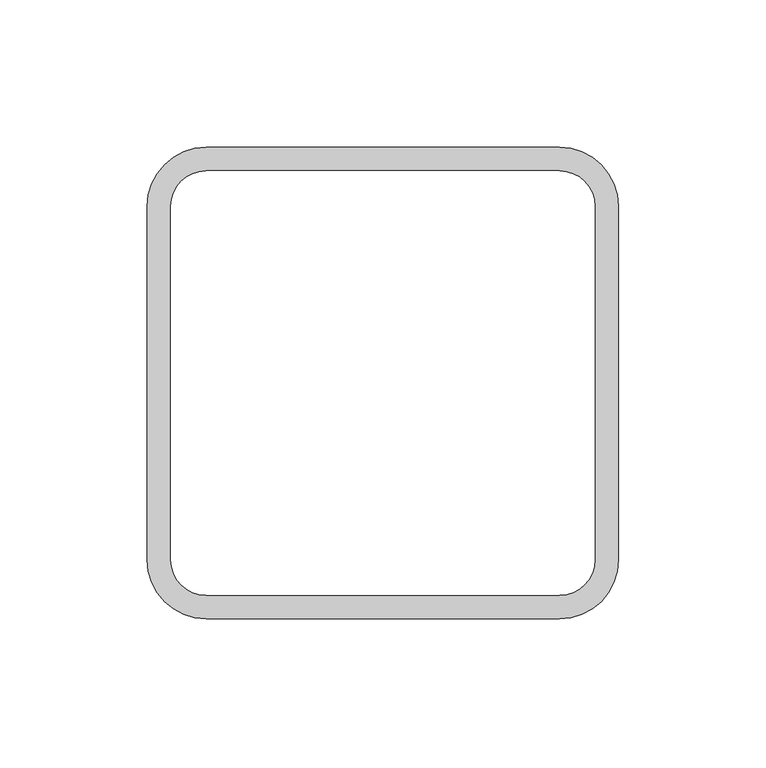
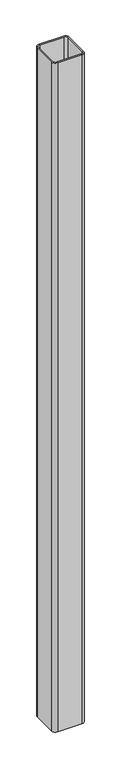
"""IFC4 building model written with IfcOpenShell, lengths in millimetres: column geometry, NLRS_28_SCO_TLB_stalen kolom buisprofiel koudgevormd vierkant-BCPG-MMBS-SRP_gen_rsf : stalen kolom buisprofiel koudgevormd vierkant RHSC_gen__160x160x8."""

import ifcopenshell
import ifcopenshell.guid

model = None  # the IFC model being written
_history = None  # IfcOwnerHistory: only IFC2X3 demands one
_inside = {}  # id of a spatial element -> (the spatial element, [elements in it])
_under = {}  # id of a project, library or spatial element -> (it, [spatial elements below it])
_declared = {}  # id of a project -> (the project, [libraries it declares])
_typed = {}  # id of a type object -> (the type object, [elements of that type])
_made_of = {}  # id of a material, layer set ... -> (it, [elements and type objects made of it])


def new_model(schema):
    """Start an empty IFC model of exactly this schema.

    Asked for "IFC4X3", IfcOpenShell would pick the latest addendum, in which some entities
    have other attributes; the version numbers below select the first issue.
    IFC2X3 requires an IfcOwnerHistory on every rooted entity: one is made here for all.
    """
    global model, _history
    if schema == "IFC4X3":
        model = ifcopenshell.file(schema_version=(4, 3, 0, 0))
    else:
        model = ifcopenshell.file(schema=schema)
    _inside.clear()
    _under.clear()
    _declared.clear()
    _typed.clear()
    _made_of.clear()
    _history = None
    if model.schema == "IFC2X3":
        org = make("IfcOrganization", Name="unknown")
        user = make(
            "IfcPersonAndOrganization",
            ThePerson=make("IfcPerson", FamilyName="unknown"),
            TheOrganization=org,
        )
        app = make(
            "IfcApplication",
            ApplicationDeveloper=org,
            Version="unknown",
            ApplicationFullName="unknown",
            ApplicationIdentifier="unknown",
        )
        _history = make(
            "IfcOwnerHistory",
            OwningUser=user,
            OwningApplication=app,
            ChangeAction="ADDED",
            CreationDate=0,
        )
    return model


def make(cls, **values):
    """One entity of the class cls with the attributes given. An attribute that is None is left unset."""
    return model.create_entity(
        cls, **{name: value for name, value in values.items() if value is not None}
    )


def rooted(cls, **values):
    """An entity with a GlobalId (a new one), such as an element, a storey or a relation."""
    return make(cls, GlobalId=ifcopenshell.guid.new(), OwnerHistory=_history, **values)


def si_unit(unit_type, name, prefix=None):
    """IfcSIUnit, for example si_unit("LENGTHUNIT", "METRE", prefix="MILLI")."""
    return make("IfcSIUnit", UnitType=unit_type, Prefix=prefix, Name=name)


def assignment(units):
    """IfcUnitAssignment: the units of a project."""
    return None if units is None else make("IfcUnitAssignment", Units=units)


def point(xyz):
    """IfcCartesianPoint."""
    return None if xyz is None else make("IfcCartesianPoint", Coordinates=xyz)


def direction(xyz):
    """IfcDirection."""
    return None if xyz is None else make("IfcDirection", DirectionRatios=xyz)


def frame(location, z_axis=None, x_axis=None):
    """IfcAxis2Placement3D, a coordinate frame: its origin and axes. An axis left out is left unset."""
    return make(
        "IfcAxis2Placement3D",
        Location=point(location),
        Axis=direction(z_axis),
        RefDirection=direction(x_axis),
    )


def frame_2d(location, x_axis=None):
    """IfcAxis2Placement2D, a coordinate frame in the plane: its origin and x axis."""
    return make(
        "IfcAxis2Placement2D", Location=point(location), RefDirection=direction(x_axis)
    )


def origin():
    """The frame at (0, 0, 0) with its axes left unset."""
    return frame((0.0, 0.0, 0.0))


def place(relative_to, where):
    """IfcLocalPlacement: puts the frame where relative to a parent placement (None: the world)."""
    return make(
        "IfcLocalPlacement", PlacementRelTo=relative_to, RelativePlacement=where
    )


def context(
    kind, dimensions, precision=None, world=None, true_north=None, identifier=None
):
    """IfcGeometricRepresentationContext, for example the 3D "Model" context."""
    return make(
        "IfcGeometricRepresentationContext",
        ContextIdentifier=identifier,
        ContextType=kind,
        CoordinateSpaceDimension=dimensions,
        Precision=precision,
        WorldCoordinateSystem=world,
        TrueNorth=true_north,
    )


def project(units=None, contexts=None):
    """IfcProject with its units and contexts."""
    return rooted(
        "IfcProject",
        Name="project",
        RepresentationContexts=contexts,
        UnitsInContext=assignment(units),
    )


def spatial(cls, under=None, at=None, **own):
    """A site, building, storey or space (cls), placed at a placement, below another one or the project."""
    s = rooted(cls, ObjectPlacement=at, **own)
    if under is not None:
        _under.setdefault(under.id(), (under, []))[1].append(s)
    return s


def polyline(points):
    """IfcPolyline through the points."""
    return make("IfcPolyline", Points=[point(p) for p in points])


def circle_curve(where, radius):
    """IfcCircle in the frame where."""
    return make("IfcCircle", Position=where, Radius=radius)


def trimmed(basis, trim1, trim2, sense, master):
    """IfcTrimmedCurve: the piece of a basis curve between two trims."""
    return make(
        "IfcTrimmedCurve",
        BasisCurve=basis,
        Trim1=trim1,
        Trim2=trim2,
        SenseAgreement=sense,
        MasterRepresentation=master,
    )


def segment(curve, same_sense, transition):
    """IfcCompositeCurveSegment."""
    return make(
        "IfcCompositeCurveSegment",
        Transition=transition,
        SameSense=same_sense,
        ParentCurve=curve,
    )


def composite_curve(segments, self_intersect=None):
    """IfcCompositeCurve: segments joined end to end."""
    return make("IfcCompositeCurve", Segments=segments, SelfIntersect=self_intersect)


def outline(outer, holes=None, kind="AREA"):
    """IfcArbitraryClosedProfileDef: a profile drawn as a closed curve; with holes, ...WithVoids."""
    if holes is None:
        return make("IfcArbitraryClosedProfileDef", ProfileType=kind, OuterCurve=outer)
    return make(
        "IfcArbitraryProfileDefWithVoids",
        ProfileType=kind,
        OuterCurve=outer,
        InnerCurves=holes,
    )


def extrude(swept, where, along, depth):
    """IfcExtrudedAreaSolid: the profile swept, set in the frame where, extruded along a direction by depth."""
    return make(
        "IfcExtrudedAreaSolid",
        SweptArea=swept,
        Position=where,
        ExtrudedDirection=direction(along),
        Depth=depth,
    )


def shape(context_of_items, identifier, shape_type, items):
    """IfcShapeRepresentation: the items that make up one representation, for example the "Body"."""
    return make(
        "IfcShapeRepresentation",
        ContextOfItems=context_of_items,
        RepresentationIdentifier=identifier,
        RepresentationType=shape_type,
        Items=items,
    )


def source(mapping_origin, context_of_items, identifier, shape_type, items):
    """IfcRepresentationMap: a shape defined once, which mapped items show again and again."""
    return make(
        "IfcRepresentationMap",
        MappingOrigin=mapping_origin,
        MappedRepresentation=shape(context_of_items, identifier, shape_type, items),
    )


def transform(
    local_origin,
    x_axis=None,
    y_axis=None,
    z_axis=None,
    scale=None,
    scale2=None,
    scale3=None,
    uniform=True,
):
    """IfcCartesianTransformationOperator3D, or its non-uniform kind. x_axis, y_axis, z_axis: its Axis1, 2, 3."""
    if uniform:
        return make(
            "IfcCartesianTransformationOperator3D",
            Axis1=direction(x_axis),
            Axis2=direction(y_axis),
            LocalOrigin=point(local_origin),
            Scale=scale,
            Axis3=direction(z_axis),
        )
    return make(
        "IfcCartesianTransformationOperator3DnonUniform",
        Axis1=direction(x_axis),
        Axis2=direction(y_axis),
        LocalOrigin=point(local_origin),
        Scale=scale,
        Axis3=direction(z_axis),
        Scale2=scale2,
        Scale3=scale3,
    )


def mapped(mapping_source, mapping_target):
    """IfcMappedItem: shows the shape of a source again, moved by a transform."""
    return make(
        "IfcMappedItem", MappingSource=mapping_source, MappingTarget=mapping_target
    )


def made_of(thing, what):
    """Note that an element or type object is made of a material, layer set ...; save() writes the relation."""
    if what is not None:
        _made_of.setdefault(what.id(), (what, []))[1].append(thing)
    return thing


def element(
    cls,
    number,
    at=None,
    inside=None,
    cuts=None,
    type_object=None,
    material=None,
    context=None,
    identifier="Body",
    shape_type=None,
    held_by="IfcProductDefinitionShape",
    body=None,
    shapes=None,
    **own,
):
    """One element of the class cls, such as IfcWall. Its Tag is "e" and its number.

    at: its placement. inside: the storey or other place that contains it. cuts: it is an
    opening in that element (IfcRelVoidsElement). A single representation is given by context,
    identifier, shape_type and body (its items); several are given by shapes. held_by: the class
    of the entity that holds the representations. save() writes the other relations.
    """
    e = rooted(cls, Tag="e%d" % number, ObjectPlacement=at, **own)
    if body is not None:
        shapes = [shape(context, identifier, shape_type, body)]
    if shapes is not None:
        e.Representation = make(held_by, Representations=shapes)
    if inside is not None:
        _inside.setdefault(inside.id(), (inside, []))[1].append(e)
    if cuts is not None:
        rooted(
            "IfcRelVoidsElement", RelatingBuildingElement=cuts, RelatedOpeningElement=e
        )
    if type_object is not None:
        _typed.setdefault(type_object.id(), (type_object, []))[1].append(e)
    return made_of(e, material)


def aggregate(whole, parts):
    """IfcRelAggregates: a whole, such as a stair, and the parts it consists of."""
    return rooted("IfcRelAggregates", RelatingObject=whole, RelatedObjects=parts)


def save(model, path):
    """Write the relations noted so far, then the file.

    IfcRelAggregates (storeys below a building ...), IfcRelContainedInSpatialStructure (elements
    in a storey), IfcRelDefinesByType, IfcRelAssociatesMaterial and IfcRelDeclares: one each for
    every whole, place, type object, material and project.
    """
    for whole, parts in _under.values():
        aggregate(whole, parts)
    for where, things in _inside.values():
        rooted(
            "IfcRelContainedInSpatialStructure",
            RelatedElements=things,
            RelatingStructure=where,
        )
    for kind, things in _typed.values():
        rooted("IfcRelDefinesByType", RelatedObjects=things, RelatingType=kind)
    for what, things in _made_of.values():
        rooted("IfcRelAssociatesMaterial", RelatedObjects=things, RelatingMaterial=what)
    for by, libraries in _declared.values():
        rooted("IfcRelDeclares", RelatingContext=by, RelatedDefinitions=libraries)
    model.write(path)


def column_9cc0dcb1(model_context):
    return source(origin(), model_context, "Body", "SweptSolid", [
        extrude(outline(composite_curve([segment(trimmed(circle_curve(frame_2d((60.0, 60.0)), 20.0), [point((60.0, 80.0))], [point((80.0, 60.0))], False, "CARTESIAN"), True, "CONTINUOUS"), segment(polyline([(80.0, 60.0), (80.0, -60.0)]), True, "CONTINUOUS"), segment(trimmed(circle_curve(frame_2d((60.0, -60.0)), 20.0), [point((80.0, -60.0))], [point((60.0, -80.0))], False, "CARTESIAN"), True, "CONTINUOUS"), segment(polyline([(60.0, -80.0), (-60.0, -80.0)]), True, "CONTINUOUS"), segment(trimmed(circle_curve(frame_2d((-60.0, -60.0)), 20.0), [point((-60.0, -80.0))], [point((-80.0, -60.0))], False, "CARTESIAN"), True, "CONTINUOUS"), segment(polyline([(-80.0, -60.0), (-80.0, 60.0)]), True, "CONTINUOUS"), segment(trimmed(circle_curve(frame_2d((-60.0, 60.0)), 20.0), [point((-80.0, 60.0))], [point((-60.0, 80.0))], False, "CARTESIAN"), True, "CONTINUOUS"), segment(polyline([(-60.0, 80.0), (60.0, 80.0)]), True, "CONTINUOUS")], self_intersect=False), holes=[composite_curve([segment(polyline([(60.0, 72.0), (-60.0, 72.0)]), True, "CONTINUOUS"), segment(trimmed(circle_curve(frame_2d((-60.0, 60.0)), 12.0), [point((-60.0, 72.0))], [point((-72.0, 60.0))], True, "CARTESIAN"), True, "CONTINUOUS"), segment(polyline([(-72.0, 60.0), (-72.0, -60.0)]), True, "CONTINUOUS"), segment(trimmed(circle_curve(frame_2d((-60.0, -60.0)), 12.0), [point((-72.0, -60.0))], [point((-60.0, -72.0))], True, "CARTESIAN"), True, "CONTINUOUS"), segment(polyline([(-60.0, -72.0), (60.0, -72.0)]), True, "CONTINUOUS"), segment(trimmed(circle_curve(frame_2d((60.0, -60.0)), 12.0), [point((60.0, -72.0))], [point((72.0, -60.0))], True, "CARTESIAN"), True, "CONTINUOUS"), segment(polyline([(72.0, -60.0), (72.0, 60.0)]), True, "CONTINUOUS"), segment(trimmed(circle_curve(frame_2d((60.0, 60.0)), 12.0), [point((72.0, 60.0))], [point((60.0, 72.0))], True, "CARTESIAN"), True, "CONTINUOUS")], self_intersect=False)]), frame((0.0, 0.0, 3760.0), z_axis=(0.0, 0.0, 1.0), x_axis=(1.0, 0.0, 0.0)), (0.0, 0.0, 1.0), 3510.0),
    ])


if __name__ == "__main__":
    model = new_model("IFC4")
    model_context = context("Model", 3, world=origin())
    ifc_project = project(units=[si_unit("LENGTHUNIT", "METRE", prefix="MILLI")], contexts=[model_context])
    site = spatial("IfcSite", under=ifc_project)
    building = spatial("IfcBuilding", under=site)
    placement = place(None, origin())
    column_shape = column_9cc0dcb1(model_context)
    element("IfcColumn", 1, ObjectType="NLRS_28_SCO_TLB_stalen kolom buisprofiel koudgevormd vierkant-BCPG-MMBS-SRP_gen_rsf : stalen kolom buisprofiel koudgevormd vierkant RHSC_gen__160x160x8", at=placement, inside=building, context=model_context, shape_type="MappedRepresentation", body=[
        mapped(column_shape, transform((0.0, 0.0, 0.0), x_axis=(1.0, 0.0, 0.0), y_axis=(0.0, 1.0, 0.0), z_axis=(0.0, 0.0, 1.0))),
    ])
    save(model, "model.ifc")

# Revit data of these elements
# Type "NLRS_28_SCO_TLB_stalen kolom buisprofiel koudgevormd vierkant-BCPG-MMBS-SRP_gen_rsf : stalen kolom buisprofiel koudgevormd vierkant RHSC_gen__160x160x8"
#   Type IfcGUID = "2$hNzCXOT3YR8V$0Cfyzxk"
#   IfcExportAs = "IfcColumnType"
#   IfcExportType = "COLUMN"
#   Type Comments = "K160x160x8"
#   Model = " "
#   Manufacturer = " "
#   Description = "stalen kolom K160x160x8"
#   Assembly Code = "28.11"
#   vz = 80 mm
#   vy = 80 mm
#   vpz = 80 mm
#   vpy = 80 mm
#   tw = 8 mm
#   tf = 8 mm
#   ri = 20 mm
#   ra = 12 mm
#   d = 160 mm
#   bf = 160 mm
#   NLRS_C_lengte [instance default] = 2743.2 mm
#   Structural Material = NLRS_h2_staal_gen_rsf
#   Keynote = ""
# Element 1 (IfcColumn, "NLRS_28_SCO_TLB_stalen kolom buisprofiel koudgevormd vierkant-BCPG-MMBS-SRP_gen_rsf : stalen kolom buisprofiel koudgevormd vierkant RHSC_gen__160x160x8")
#   NLRS_C_lengte = 3510 mm
#   Materials on its faces: "NLRS_h2_staal_gen_rsf"
# Materials
#   "NLRS_h2_staal_gen_rsf": class "H - Metaal", colour RGB 189 187 185, transparency 0, Keynote = "h2", Manufacturer = "Revit Standards Foundation", URL = "www.revitstandards.org", Description = "staal", Cost = 0
